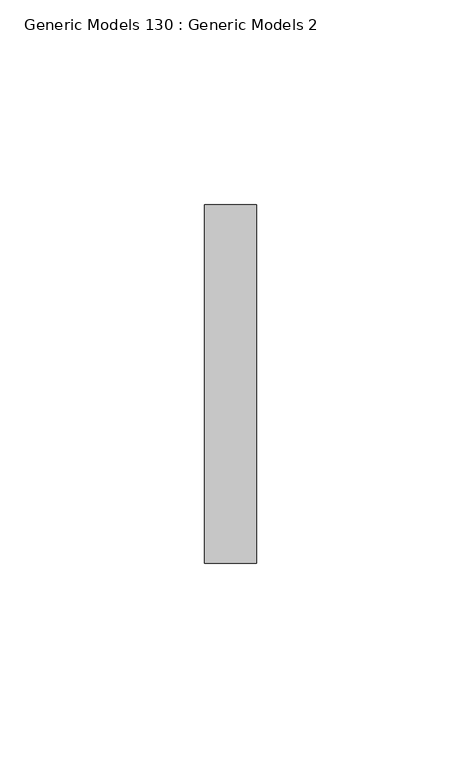
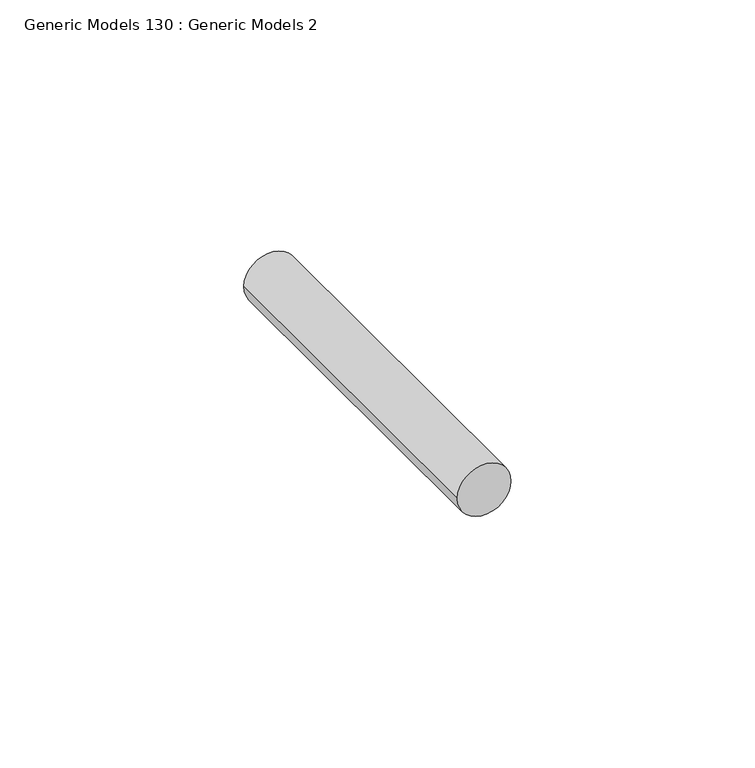
"""IFC4 building model written with IfcOpenShell, lengths in millimetres: proxy geometry, Generic Models 130 : Generic Models 2."""

from ifc_helpers import new_model, si_unit, point, frame, frame_2d, origin, place, context, project, spatial, circle_curve, trimmed, segment, composite_curve, outline, extrude, source, transform, mapped, element, save


def generic_models_130_generic_models_2_0c7de630(model_context):
    return source(origin(), model_context, "Body", "SweptSolid", [
        extrude(outline(composite_curve([segment(trimmed(circle_curve(frame_2d((38546.4677238, 7966.3828124)), 6.35), [point((38546.4677238, 7960.0328124))], [point((38546.4677238, 7972.7328124))], False, "CARTESIAN"), True, "CONTINUOUS"), segment(trimmed(circle_curve(frame_2d((38546.4677238, 7966.3828124)), 6.35), [point((38546.4677238, 7972.7328124))], [point((38546.4677238, 7960.0328124))], False, "CARTESIAN"), True, "CONTINUOUS")], self_intersect=False)), frame((0.0, 1848.3666731, 0.0), z_axis=(0.0, 1.0, 0.0), x_axis=(0.0, 0.0, 1.0)), (0.0, 0.0, 1.0), 87.551022),
    ])


if __name__ == "__main__":
    model = new_model("IFC4")
    model_context = context("Model", 3, world=origin())
    ifc_project = project(units=[si_unit("LENGTHUNIT", "METRE", prefix="MILLI")], contexts=[model_context])
    site = spatial("IfcSite", under=ifc_project)
    building = spatial("IfcBuilding", under=site)
    placement = place(None, origin())
    generic_models_130_generic_models_2_shape = generic_models_130_generic_models_2_0c7de630(model_context)
    element("IfcBuildingElementProxy", 1, Name="Generic Models 130 : Generic Models 2", ObjectType="Generic Models 130 : Generic Models 2", at=placement, inside=building, context=model_context, shape_type="MappedRepresentation", body=[
        mapped(generic_models_130_generic_models_2_shape, transform((0.0, 0.0, 0.0), x_axis=(1.0, 0.0, 0.0), y_axis=(0.0, 1.0, 0.0), z_axis=(0.0, 0.0, 1.0))),
    ])
    save(model, "model.ifc")

# Revit data of these elements
# Element 1 (IfcBuildingElementProxy, "Generic Models 130 : Generic Models 2")
#   Materials on its faces: "S.S. LAG BOLT - SEE STRUCT. DWGS"
# Materials
#   "S.S. LAG BOLT - SEE STRUCT. DWGS": class "Generic", colour RGB 120 120 120, transparency 0, Cost = 0
